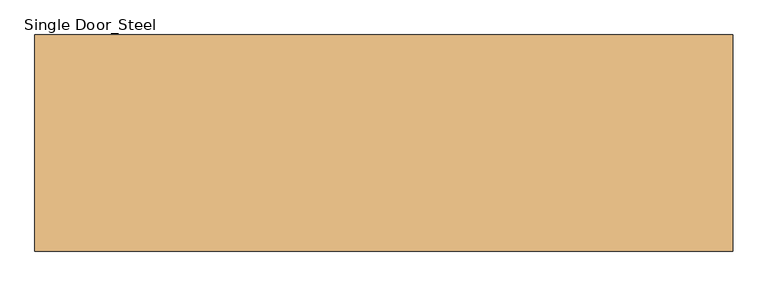
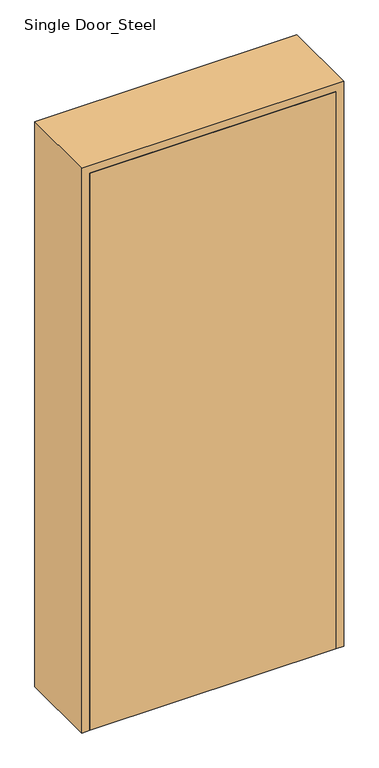
"""IFC4 building model written with IfcOpenShell, lengths in millimetres: door geometry, Single Door_Steel : H_DR_AR_B12_Single Door_Steel_W1000xH2280_FSD1."""

import ifcopenshell
import ifcopenshell.guid

model = None  # the IFC model being written
_history = None  # IfcOwnerHistory: only IFC2X3 demands one
_inside = {}  # id of a spatial element -> (the spatial element, [elements in it])
_under = {}  # id of a project, library or spatial element -> (it, [spatial elements below it])
_declared = {}  # id of a project -> (the project, [libraries it declares])
_typed = {}  # id of a type object -> (the type object, [elements of that type])
_made_of = {}  # id of a material, layer set ... -> (it, [elements and type objects made of it])


def new_model(schema):
    """Start an empty IFC model of exactly this schema.

    Asked for "IFC4X3", IfcOpenShell would pick the latest addendum, in which some entities
    have other attributes; the version numbers below select the first issue.
    IFC2X3 requires an IfcOwnerHistory on every rooted entity: one is made here for all.
    """
    global model, _history
    if schema == "IFC4X3":
        model = ifcopenshell.file(schema_version=(4, 3, 0, 0))
    else:
        model = ifcopenshell.file(schema=schema)
    _inside.clear()
    _under.clear()
    _declared.clear()
    _typed.clear()
    _made_of.clear()
    _history = None
    if model.schema == "IFC2X3":
        org = make("IfcOrganization", Name="unknown")
        user = make(
            "IfcPersonAndOrganization",
            ThePerson=make("IfcPerson", FamilyName="unknown"),
            TheOrganization=org,
        )
        app = make(
            "IfcApplication",
            ApplicationDeveloper=org,
            Version="unknown",
            ApplicationFullName="unknown",
            ApplicationIdentifier="unknown",
        )
        _history = make(
            "IfcOwnerHistory",
            OwningUser=user,
            OwningApplication=app,
            ChangeAction="ADDED",
            CreationDate=0,
        )
    return model


def make(cls, **values):
    """One entity of the class cls with the attributes given. An attribute that is None is left unset."""
    return model.create_entity(
        cls, **{name: value for name, value in values.items() if value is not None}
    )


def rooted(cls, **values):
    """An entity with a GlobalId (a new one), such as an element, a storey or a relation."""
    return make(cls, GlobalId=ifcopenshell.guid.new(), OwnerHistory=_history, **values)


def si_unit(unit_type, name, prefix=None):
    """IfcSIUnit, for example si_unit("LENGTHUNIT", "METRE", prefix="MILLI")."""
    return make("IfcSIUnit", UnitType=unit_type, Prefix=prefix, Name=name)


def assignment(units):
    """IfcUnitAssignment: the units of a project."""
    return None if units is None else make("IfcUnitAssignment", Units=units)


def point(xyz):
    """IfcCartesianPoint."""
    return None if xyz is None else make("IfcCartesianPoint", Coordinates=xyz)


def direction(xyz):
    """IfcDirection."""
    return None if xyz is None else make("IfcDirection", DirectionRatios=xyz)


def frame(location, z_axis=None, x_axis=None):
    """IfcAxis2Placement3D, a coordinate frame: its origin and axes. An axis left out is left unset."""
    return make(
        "IfcAxis2Placement3D",
        Location=point(location),
        Axis=direction(z_axis),
        RefDirection=direction(x_axis),
    )


def origin():
    """The frame at (0, 0, 0) with its axes left unset."""
    return frame((0.0, 0.0, 0.0))


def origin_with_axes():
    """The frame at (0, 0, 0) with the z axis (0, 0, 1) and the x axis (1, 0, 0) written out."""
    return frame((0.0, 0.0, 0.0), z_axis=(0.0, 0.0, 1.0), x_axis=(1.0, 0.0, 0.0))


def place(relative_to, where):
    """IfcLocalPlacement: puts the frame where relative to a parent placement (None: the world)."""
    return make(
        "IfcLocalPlacement", PlacementRelTo=relative_to, RelativePlacement=where
    )


def context(
    kind, dimensions, precision=None, world=None, true_north=None, identifier=None
):
    """IfcGeometricRepresentationContext, for example the 3D "Model" context."""
    return make(
        "IfcGeometricRepresentationContext",
        ContextIdentifier=identifier,
        ContextType=kind,
        CoordinateSpaceDimension=dimensions,
        Precision=precision,
        WorldCoordinateSystem=world,
        TrueNorth=true_north,
    )


def project(units=None, contexts=None):
    """IfcProject with its units and contexts."""
    return rooted(
        "IfcProject",
        Name="project",
        RepresentationContexts=contexts,
        UnitsInContext=assignment(units),
    )


def spatial(cls, under=None, at=None, **own):
    """A site, building, storey or space (cls), placed at a placement, below another one or the project."""
    s = rooted(cls, ObjectPlacement=at, **own)
    if under is not None:
        _under.setdefault(under.id(), (under, []))[1].append(s)
    return s


def polyline(points):
    """IfcPolyline through the points."""
    return make("IfcPolyline", Points=[point(p) for p in points])


def outline(outer, holes=None, kind="AREA"):
    """IfcArbitraryClosedProfileDef: a profile drawn as a closed curve; with holes, ...WithVoids."""
    if holes is None:
        return make("IfcArbitraryClosedProfileDef", ProfileType=kind, OuterCurve=outer)
    return make(
        "IfcArbitraryProfileDefWithVoids",
        ProfileType=kind,
        OuterCurve=outer,
        InnerCurves=holes,
    )


def extrude(swept, where, along, depth):
    """IfcExtrudedAreaSolid: the profile swept, set in the frame where, extruded along a direction by depth."""
    return make(
        "IfcExtrudedAreaSolid",
        SweptArea=swept,
        Position=where,
        ExtrudedDirection=direction(along),
        Depth=depth,
    )


def faces_of(points, faces, orient=None, outer=None):
    """IfcFace entities. A face is a list of loops; a loop is a list of indices into points, from 0.

    orient and outer hold one flag for each loop. By default every Orientation is true, the
    first loop of a face is its IfcFaceOuterBound and the others are IfcFaceBound.
    """
    made = []
    for i, loops in enumerate(faces):
        bounds = []
        for j, loop in enumerate(loops):
            is_outer = j == 0 if outer is None else outer[i][j]
            bounds.append(
                make(
                    "IfcFaceOuterBound" if is_outer else "IfcFaceBound",
                    Bound=make("IfcPolyLoop", Polygon=[points[k] for k in loop]),
                    Orientation=True if orient is None else orient[i][j],
                )
            )
        made.append(make("IfcFace", Bounds=bounds))
    return made


def faceted_brep(points, faces, orient=None, outer=None, voids=None):
    """IfcFacetedBrep: a solid bounded by flat faces; with voids (closed shells), ...WithVoids."""
    shared = [point(p) for p in points]
    hull = make("IfcClosedShell", CfsFaces=faces_of(shared, faces, orient, outer))
    if voids is None:
        return make("IfcFacetedBrep", Outer=hull)
    return make(
        "IfcFacetedBrepWithVoids",
        Outer=hull,
        Voids=[
            make(cls, CfsFaces=faces_of(shared, fs, o, b)) for cls, fs, o, b in voids
        ],
    )


def shape(context_of_items, identifier, shape_type, items):
    """IfcShapeRepresentation: the items that make up one representation, for example the "Body"."""
    return make(
        "IfcShapeRepresentation",
        ContextOfItems=context_of_items,
        RepresentationIdentifier=identifier,
        RepresentationType=shape_type,
        Items=items,
    )


def source(mapping_origin, context_of_items, identifier, shape_type, items):
    """IfcRepresentationMap: a shape defined once, which mapped items show again and again."""
    return make(
        "IfcRepresentationMap",
        MappingOrigin=mapping_origin,
        MappedRepresentation=shape(context_of_items, identifier, shape_type, items),
    )


def transform(
    local_origin,
    x_axis=None,
    y_axis=None,
    z_axis=None,
    scale=None,
    scale2=None,
    scale3=None,
    uniform=True,
):
    """IfcCartesianTransformationOperator3D, or its non-uniform kind. x_axis, y_axis, z_axis: its Axis1, 2, 3."""
    if uniform:
        return make(
            "IfcCartesianTransformationOperator3D",
            Axis1=direction(x_axis),
            Axis2=direction(y_axis),
            LocalOrigin=point(local_origin),
            Scale=scale,
            Axis3=direction(z_axis),
        )
    return make(
        "IfcCartesianTransformationOperator3DnonUniform",
        Axis1=direction(x_axis),
        Axis2=direction(y_axis),
        LocalOrigin=point(local_origin),
        Scale=scale,
        Axis3=direction(z_axis),
        Scale2=scale2,
        Scale3=scale3,
    )


def mapped(mapping_source, mapping_target):
    """IfcMappedItem: shows the shape of a source again, moved by a transform."""
    return make(
        "IfcMappedItem", MappingSource=mapping_source, MappingTarget=mapping_target
    )


def made_of(thing, what):
    """Note that an element or type object is made of a material, layer set ...; save() writes the relation."""
    if what is not None:
        _made_of.setdefault(what.id(), (what, []))[1].append(thing)
    return thing


def element(
    cls,
    number,
    at=None,
    inside=None,
    cuts=None,
    type_object=None,
    material=None,
    context=None,
    identifier="Body",
    shape_type=None,
    held_by="IfcProductDefinitionShape",
    body=None,
    shapes=None,
    **own,
):
    """One element of the class cls, such as IfcWall. Its Tag is "e" and its number.

    at: its placement. inside: the storey or other place that contains it. cuts: it is an
    opening in that element (IfcRelVoidsElement). A single representation is given by context,
    identifier, shape_type and body (its items); several are given by shapes. held_by: the class
    of the entity that holds the representations. save() writes the other relations.
    """
    e = rooted(cls, Tag="e%d" % number, ObjectPlacement=at, **own)
    if body is not None:
        shapes = [shape(context, identifier, shape_type, body)]
    if shapes is not None:
        e.Representation = make(held_by, Representations=shapes)
    if inside is not None:
        _inside.setdefault(inside.id(), (inside, []))[1].append(e)
    if cuts is not None:
        rooted(
            "IfcRelVoidsElement", RelatingBuildingElement=cuts, RelatedOpeningElement=e
        )
    if type_object is not None:
        _typed.setdefault(type_object.id(), (type_object, []))[1].append(e)
    return made_of(e, material)


def aggregate(whole, parts):
    """IfcRelAggregates: a whole, such as a stair, and the parts it consists of."""
    return rooted("IfcRelAggregates", RelatingObject=whole, RelatedObjects=parts)


def save(model, path):
    """Write the relations noted so far, then the file.

    IfcRelAggregates (storeys below a building ...), IfcRelContainedInSpatialStructure (elements
    in a storey), IfcRelDefinesByType, IfcRelAssociatesMaterial and IfcRelDeclares: one each for
    every whole, place, type object, material and project.
    """
    for whole, parts in _under.values():
        aggregate(whole, parts)
    for where, things in _inside.values():
        rooted(
            "IfcRelContainedInSpatialStructure",
            RelatedElements=things,
            RelatingStructure=where,
        )
    for kind, things in _typed.values():
        rooted("IfcRelDefinesByType", RelatedObjects=things, RelatingType=kind)
    for what, things in _made_of.values():
        rooted("IfcRelAssociatesMaterial", RelatedObjects=things, RelatingMaterial=what)
    for by, libraries in _declared.values():
        rooted("IfcRelDeclares", RelatingContext=by, RelatedDefinitions=libraries)
    model.write(path)


def single_door_steel_001f4ee4(model_context):
    return source(origin(), model_context, "Body", "SolidModel", [
        extrude(outline(polyline([(470.0, -155.0), (-470.0, -155.0), (-470.0, -120.0), (470.0, -120.0), (470.0, -155.0)])), origin_with_axes(), (0.0, 0.0, 1.0), 2250.0),
        faceted_brep([(470.0, -155.0, 0.0), (470.0, -120.0, 0.0), (450.0, -120.0, 0.0), (450.0, 120.0, 0.0), (470.0, 120.0, 0.0), (470.0, 155.0, 0.0), (500.0, 155.0, 0.0), (500.0, -155.0, 0.0), (500.0, -155.0, 2280.0), (-500.0, -155.0, 2280.0), (-500.0, -155.0, 0.0), (-470.0, -155.0, 0.0), (-470.0, -155.0, 2250.0), (470.0, -155.0, 2250.0), (500.0, 155.0, 2280.0), (470.0, 155.0, 2250.0), (-470.0, 155.0, 2250.0), (-470.0, 155.0, 0.0), (-500.0, 155.0, 0.0), (-500.0, 155.0, 2280.0), (470.0, 120.0, 2250.0), (450.0, 120.0, 2230.0), (-450.0, 120.0, 2230.0), (-450.0, 120.0, 0.0), (-470.0, 120.0, 0.0), (-470.0, 120.0, 2250.0), (450.0, -120.0, 2230.0), (470.0, -120.0, 2250.0), (-470.0, -120.0, 2250.0), (-470.0, -120.0, 0.0), (-450.0, -120.0, 0.0), (-450.0, -120.0, 2230.0)], [[[0, 1, 2, 3, 4, 5, 6, 7]], [[7, 8, 9, 10, 11, 12, 13, 0]], [[6, 14, 8, 7]], [[5, 15, 16, 17, 18, 19, 14, 6]], [[4, 20, 15, 5]], [[3, 21, 22, 23, 24, 25, 20, 4]], [[2, 26, 21, 3]], [[1, 27, 28, 29, 30, 31, 26, 2]], [[0, 13, 27, 1]], [[12, 11, 29, 28]], [[11, 10, 18, 17, 24, 23, 30, 29]], [[19, 18, 10, 9]], [[25, 24, 17, 16]], [[31, 30, 23, 22]], [[14, 19, 9, 8]], [[20, 25, 16, 15]], [[26, 31, 22, 21]], [[13, 12, 28, 27]]]),
    ])


if __name__ == "__main__":
    model = new_model("IFC4")
    model_context = context("Model", 3, world=origin())
    ifc_project = project(units=[si_unit("LENGTHUNIT", "METRE", prefix="MILLI")], contexts=[model_context])
    site = spatial("IfcSite", under=ifc_project)
    building = spatial("IfcBuilding", under=site)
    placement = place(None, origin())
    single_door_steel_shape = single_door_steel_001f4ee4(model_context)
    element("IfcDoor", 1, ObjectType="Single Door_Steel : H_DR_AR_B12_Single Door_Steel_W1000xH2280_FSD1", at=placement, inside=building, context=model_context, shape_type="MappedRepresentation", body=[
        mapped(single_door_steel_shape, transform((0.0, 0.0, 0.0), x_axis=(1.0, 0.0, 0.0), y_axis=(0.0, 1.0, 0.0), z_axis=(0.0, 0.0, 1.0))),
    ])
    save(model, "model.ifc")

# Revit data of these elements
# Type "Single Door_Steel : H_DR_AR_B12_Single Door_Steel_W1000xH2280_FSD1"
#   Type Mark = "439"
#   Analytic Construction = "<None>"
#   프레임 투영 외부. = 25 mm
#   프레임 투영 내부. = 25 mm
#   프레임 폭 = 75 mm
#   Height = 2280 mm
#   Width = 1000 mm
#   Define Thermal Properties by = 1
#   문 패널 = none
#   문 프레임 = none
#   Function = (empty or 0)
#   Wall Closure = (empty or 0)
